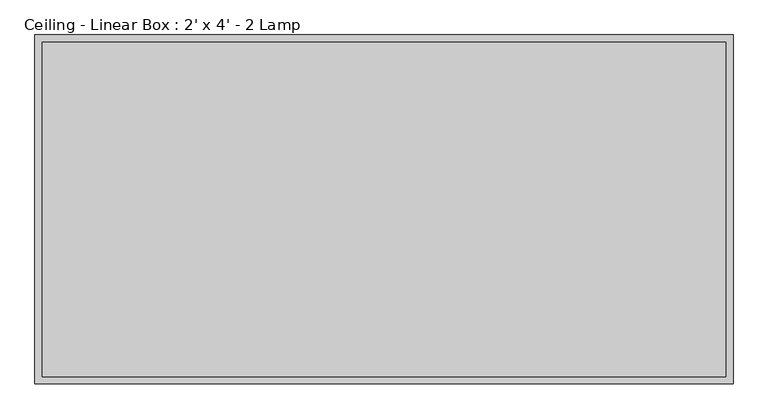
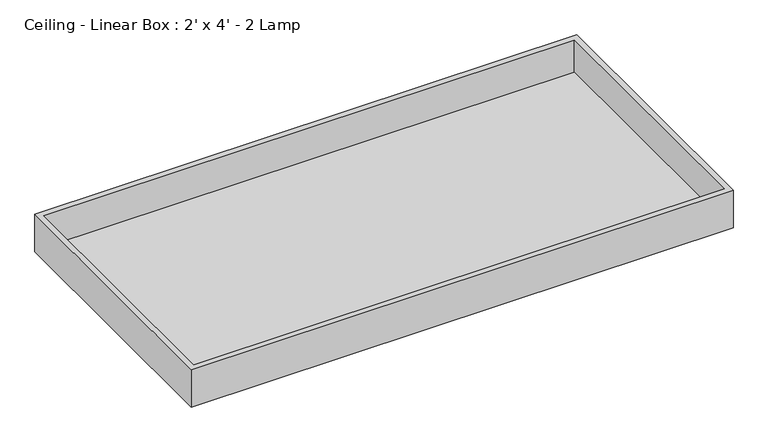
"""IFC4 building model written with IfcOpenShell, lengths in millimetres: light fixture geometry, Ceiling - Linear Box : 2' x 4' - 2 Lamp."""

from ifc_helpers import new_model, si_unit, frame, origin, place, context, project, spatial, polyline, outline, extrude, source, transform, mapped, element, save


def ceiling_linear_box_2_x_4_2_lamp_6471e3e8(model_context):
    return source(origin(), model_context, "Body", "SweptSolid", [
        extrude(outline(polyline([(596.9, 292.1), (596.9, -292.1), (-596.9, -292.1), (-596.9, 292.1), (596.9, 292.1)])), frame((0.0, 0.0, 2355.85), z_axis=(0.0, 0.0, 1.0), x_axis=(1.0, 0.0, 0.0)), (0.0, 0.0, 1.0), 6.35),
        extrude(outline(polyline([(609.6, 304.8), (609.6, -304.8), (-609.6, -304.8), (-609.6, 304.8), (609.6, 304.8)]), holes=[polyline([(596.9, 292.1), (-596.9, 292.1), (-596.9, -292.1), (596.9, -292.1), (596.9, 292.1)])]), frame((0.0, 0.0, 2349.5), z_axis=(0.0, 0.0, 1.0), x_axis=(1.0, 0.0, 0.0)), (0.0, 0.0, 1.0), 88.9),
    ])


if __name__ == "__main__":
    model = new_model("IFC4")
    model_context = context("Model", 3, world=origin())
    ifc_project = project(units=[si_unit("LENGTHUNIT", "METRE", prefix="MILLI")], contexts=[model_context])
    site = spatial("IfcSite", under=ifc_project)
    building = spatial("IfcBuilding", under=site)
    placement = place(None, origin())
    ceiling_linear_box_2_x_4_2_lamp_shape = ceiling_linear_box_2_x_4_2_lamp_6471e3e8(model_context)
    element("IfcLightFixture", 1, ObjectType="Ceiling - Linear Box : 2' x 4' - 2 Lamp", at=placement, inside=building, context=model_context, shape_type="MappedRepresentation", body=[
        mapped(ceiling_linear_box_2_x_4_2_lamp_shape, transform((0.0, 0.0, 0.0), x_axis=(1.0, 0.0, 0.0), y_axis=(0.0, 1.0, 0.0), z_axis=(0.0, 0.0, 1.0))),
    ])
    save(model, "model.ifc")

# Revit data of these elements
# Type "Ceiling - Linear Box : 2' x 4' - 2 Lamp"
#   Assembly Code = "D5020210"
#   Lamp = "T-12"
#   Wattage = 32.3141 W
#   built-in parameter 1150110 = 1 (stored number, unit not read)
#   built-in parameter 1114217 = 1 (stored number, unit not read)
#   built-in parameter 1150109 = 1 (stored number, unit not read)
#   built-in parameter 1150113 = 1 (stored number, unit not read)
#   built-in parameter 1150105 = 381.972 (stored number, unit not read)
#   built-in parameter 1150115 = 1 (stored number, unit not read)
#   Light Source Symbol Size = 2' - 0"
#   built-in parameter 1150112 = 1 (stored number, unit not read)
#   built-in parameter 1150114 = 1 (stored number, unit not read)
#   built-in parameter 1150107 = 3200 (stored number, unit not read)
#   built-in parameter 1150106 = 3.81972 (stored number, unit not read)
#   Emit from Line Length = 2' - 0"
#   built-in parameter 1150104 = 13.8 (stored number, unit not read)
#   built-in parameter 1114218 = 1 (stored number, unit not read)
#   built-in parameter 1150133 = 10 (stored number, unit not read)
#   Length = 4' - 0"
#   Lumens = 4800 lm
#   Width = 2' - 0"
#   built-in parameter 1150134 = 3
#   built-in parameter 1150132 = 2
#   Color Filter = 16777215
#   Diffuser = none
#   Light Box = none
#   Dimming Lamp Color Temperature Shift = (empty or 0)
